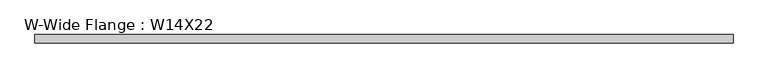
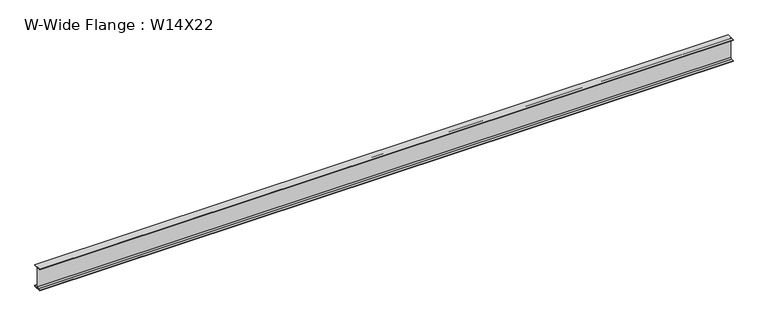
"""IFC4 building model written with IfcOpenShell, lengths in millimetres: beam geometry, W-Wide Flange : W14X22."""

import ifcopenshell
import ifcopenshell.guid

model = None  # the IFC model being written
_history = None  # IfcOwnerHistory: only IFC2X3 demands one
_inside = {}  # id of a spatial element -> (the spatial element, [elements in it])
_under = {}  # id of a project, library or spatial element -> (it, [spatial elements below it])
_declared = {}  # id of a project -> (the project, [libraries it declares])
_typed = {}  # id of a type object -> (the type object, [elements of that type])
_made_of = {}  # id of a material, layer set ... -> (it, [elements and type objects made of it])


def new_model(schema):
    """Start an empty IFC model of exactly this schema.

    Asked for "IFC4X3", IfcOpenShell would pick the latest addendum, in which some entities
    have other attributes; the version numbers below select the first issue.
    IFC2X3 requires an IfcOwnerHistory on every rooted entity: one is made here for all.
    """
    global model, _history
    if schema == "IFC4X3":
        model = ifcopenshell.file(schema_version=(4, 3, 0, 0))
    else:
        model = ifcopenshell.file(schema=schema)
    _inside.clear()
    _under.clear()
    _declared.clear()
    _typed.clear()
    _made_of.clear()
    _history = None
    if model.schema == "IFC2X3":
        org = make("IfcOrganization", Name="unknown")
        user = make(
            "IfcPersonAndOrganization",
            ThePerson=make("IfcPerson", FamilyName="unknown"),
            TheOrganization=org,
        )
        app = make(
            "IfcApplication",
            ApplicationDeveloper=org,
            Version="unknown",
            ApplicationFullName="unknown",
            ApplicationIdentifier="unknown",
        )
        _history = make(
            "IfcOwnerHistory",
            OwningUser=user,
            OwningApplication=app,
            ChangeAction="ADDED",
            CreationDate=0,
        )
    return model


def make(cls, **values):
    """One entity of the class cls with the attributes given. An attribute that is None is left unset."""
    return model.create_entity(
        cls, **{name: value for name, value in values.items() if value is not None}
    )


def rooted(cls, **values):
    """An entity with a GlobalId (a new one), such as an element, a storey or a relation."""
    return make(cls, GlobalId=ifcopenshell.guid.new(), OwnerHistory=_history, **values)


def si_unit(unit_type, name, prefix=None):
    """IfcSIUnit, for example si_unit("LENGTHUNIT", "METRE", prefix="MILLI")."""
    return make("IfcSIUnit", UnitType=unit_type, Prefix=prefix, Name=name)


def assignment(units):
    """IfcUnitAssignment: the units of a project."""
    return None if units is None else make("IfcUnitAssignment", Units=units)


def point(xyz):
    """IfcCartesianPoint."""
    return None if xyz is None else make("IfcCartesianPoint", Coordinates=xyz)


def direction(xyz):
    """IfcDirection."""
    return None if xyz is None else make("IfcDirection", DirectionRatios=xyz)


def frame(location, z_axis=None, x_axis=None):
    """IfcAxis2Placement3D, a coordinate frame: its origin and axes. An axis left out is left unset."""
    return make(
        "IfcAxis2Placement3D",
        Location=point(location),
        Axis=direction(z_axis),
        RefDirection=direction(x_axis),
    )


def frame_2d(location, x_axis=None):
    """IfcAxis2Placement2D, a coordinate frame in the plane: its origin and x axis."""
    return make(
        "IfcAxis2Placement2D", Location=point(location), RefDirection=direction(x_axis)
    )


def origin():
    """The frame at (0, 0, 0) with its axes left unset."""
    return frame((0.0, 0.0, 0.0))


def place(relative_to, where):
    """IfcLocalPlacement: puts the frame where relative to a parent placement (None: the world)."""
    return make(
        "IfcLocalPlacement", PlacementRelTo=relative_to, RelativePlacement=where
    )


def context(
    kind, dimensions, precision=None, world=None, true_north=None, identifier=None
):
    """IfcGeometricRepresentationContext, for example the 3D "Model" context."""
    return make(
        "IfcGeometricRepresentationContext",
        ContextIdentifier=identifier,
        ContextType=kind,
        CoordinateSpaceDimension=dimensions,
        Precision=precision,
        WorldCoordinateSystem=world,
        TrueNorth=true_north,
    )


def project(units=None, contexts=None):
    """IfcProject with its units and contexts."""
    return rooted(
        "IfcProject",
        Name="project",
        RepresentationContexts=contexts,
        UnitsInContext=assignment(units),
    )


def spatial(cls, under=None, at=None, **own):
    """A site, building, storey or space (cls), placed at a placement, below another one or the project."""
    s = rooted(cls, ObjectPlacement=at, **own)
    if under is not None:
        _under.setdefault(under.id(), (under, []))[1].append(s)
    return s


def polyline(points):
    """IfcPolyline through the points."""
    return make("IfcPolyline", Points=[point(p) for p in points])


def circle_curve(where, radius):
    """IfcCircle in the frame where."""
    return make("IfcCircle", Position=where, Radius=radius)


def trimmed(basis, trim1, trim2, sense, master):
    """IfcTrimmedCurve: the piece of a basis curve between two trims."""
    return make(
        "IfcTrimmedCurve",
        BasisCurve=basis,
        Trim1=trim1,
        Trim2=trim2,
        SenseAgreement=sense,
        MasterRepresentation=master,
    )


def segment(curve, same_sense, transition):
    """IfcCompositeCurveSegment."""
    return make(
        "IfcCompositeCurveSegment",
        Transition=transition,
        SameSense=same_sense,
        ParentCurve=curve,
    )


def composite_curve(segments, self_intersect=None):
    """IfcCompositeCurve: segments joined end to end."""
    return make("IfcCompositeCurve", Segments=segments, SelfIntersect=self_intersect)


def outline(outer, holes=None, kind="AREA"):
    """IfcArbitraryClosedProfileDef: a profile drawn as a closed curve; with holes, ...WithVoids."""
    if holes is None:
        return make("IfcArbitraryClosedProfileDef", ProfileType=kind, OuterCurve=outer)
    return make(
        "IfcArbitraryProfileDefWithVoids",
        ProfileType=kind,
        OuterCurve=outer,
        InnerCurves=holes,
    )


def extrude(swept, where, along, depth):
    """IfcExtrudedAreaSolid: the profile swept, set in the frame where, extruded along a direction by depth."""
    return make(
        "IfcExtrudedAreaSolid",
        SweptArea=swept,
        Position=where,
        ExtrudedDirection=direction(along),
        Depth=depth,
    )


def shape(context_of_items, identifier, shape_type, items):
    """IfcShapeRepresentation: the items that make up one representation, for example the "Body"."""
    return make(
        "IfcShapeRepresentation",
        ContextOfItems=context_of_items,
        RepresentationIdentifier=identifier,
        RepresentationType=shape_type,
        Items=items,
    )


def source(mapping_origin, context_of_items, identifier, shape_type, items):
    """IfcRepresentationMap: a shape defined once, which mapped items show again and again."""
    return make(
        "IfcRepresentationMap",
        MappingOrigin=mapping_origin,
        MappedRepresentation=shape(context_of_items, identifier, shape_type, items),
    )


def transform(
    local_origin,
    x_axis=None,
    y_axis=None,
    z_axis=None,
    scale=None,
    scale2=None,
    scale3=None,
    uniform=True,
):
    """IfcCartesianTransformationOperator3D, or its non-uniform kind. x_axis, y_axis, z_axis: its Axis1, 2, 3."""
    if uniform:
        return make(
            "IfcCartesianTransformationOperator3D",
            Axis1=direction(x_axis),
            Axis2=direction(y_axis),
            LocalOrigin=point(local_origin),
            Scale=scale,
            Axis3=direction(z_axis),
        )
    return make(
        "IfcCartesianTransformationOperator3DnonUniform",
        Axis1=direction(x_axis),
        Axis2=direction(y_axis),
        LocalOrigin=point(local_origin),
        Scale=scale,
        Axis3=direction(z_axis),
        Scale2=scale2,
        Scale3=scale3,
    )


def mapped(mapping_source, mapping_target):
    """IfcMappedItem: shows the shape of a source again, moved by a transform."""
    return make(
        "IfcMappedItem", MappingSource=mapping_source, MappingTarget=mapping_target
    )


def made_of(thing, what):
    """Note that an element or type object is made of a material, layer set ...; save() writes the relation."""
    if what is not None:
        _made_of.setdefault(what.id(), (what, []))[1].append(thing)
    return thing


def element(
    cls,
    number,
    at=None,
    inside=None,
    cuts=None,
    type_object=None,
    material=None,
    context=None,
    identifier="Body",
    shape_type=None,
    held_by="IfcProductDefinitionShape",
    body=None,
    shapes=None,
    **own,
):
    """One element of the class cls, such as IfcWall. Its Tag is "e" and its number.

    at: its placement. inside: the storey or other place that contains it. cuts: it is an
    opening in that element (IfcRelVoidsElement). A single representation is given by context,
    identifier, shape_type and body (its items); several are given by shapes. held_by: the class
    of the entity that holds the representations. save() writes the other relations.
    """
    e = rooted(cls, Tag="e%d" % number, ObjectPlacement=at, **own)
    if body is not None:
        shapes = [shape(context, identifier, shape_type, body)]
    if shapes is not None:
        e.Representation = make(held_by, Representations=shapes)
    if inside is not None:
        _inside.setdefault(inside.id(), (inside, []))[1].append(e)
    if cuts is not None:
        rooted(
            "IfcRelVoidsElement", RelatingBuildingElement=cuts, RelatedOpeningElement=e
        )
    if type_object is not None:
        _typed.setdefault(type_object.id(), (type_object, []))[1].append(e)
    return made_of(e, material)


def aggregate(whole, parts):
    """IfcRelAggregates: a whole, such as a stair, and the parts it consists of."""
    return rooted("IfcRelAggregates", RelatingObject=whole, RelatedObjects=parts)


def save(model, path):
    """Write the relations noted so far, then the file.

    IfcRelAggregates (storeys below a building ...), IfcRelContainedInSpatialStructure (elements
    in a storey), IfcRelDefinesByType, IfcRelAssociatesMaterial and IfcRelDeclares: one each for
    every whole, place, type object, material and project.
    """
    for whole, parts in _under.values():
        aggregate(whole, parts)
    for where, things in _inside.values():
        rooted(
            "IfcRelContainedInSpatialStructure",
            RelatedElements=things,
            RelatingStructure=where,
        )
    for kind, things in _typed.values():
        rooted("IfcRelDefinesByType", RelatedObjects=things, RelatingType=kind)
    for what, things in _made_of.values():
        rooted("IfcRelAssociatesMaterial", RelatedObjects=things, RelatingMaterial=what)
    for by, libraries in _declared.values():
        rooted("IfcRelDeclares", RelatingContext=by, RelatedDefinitions=libraries)
    model.write(path)


def w_wide_flange_w14x22_9d42d0bf(model_context):
    return source(origin(), model_context, "Body", "SweptSolid", [
        extrude(outline(composite_curve([segment(polyline([(63.5, -165.481), (63.5, -173.99), (-63.5, -173.99), (-63.5, -165.481), (-21.3995, -165.481)]), True, "CONTINUOUS"), segment(trimmed(circle_curve(frame_2d((-21.3995, -147.0025)), 18.4785), [point((-21.3995, -165.481))], [point((-2.921, -147.0025))], True, "CARTESIAN"), True, "CONTINUOUS"), segment(polyline([(-2.921, -147.0025), (-2.921, 147.0025)]), True, "CONTINUOUS"), segment(trimmed(circle_curve(frame_2d((-21.3995, 147.0025)), 18.4785), [point((-2.921, 147.0025))], [point((-21.3995, 165.481))], True, "CARTESIAN"), True, "CONTINUOUS"), segment(polyline([(-21.3995, 165.481), (-63.5, 165.481), (-63.5, 173.99), (63.5, 173.99), (63.5, 165.481), (21.3995, 165.481)]), True, "CONTINUOUS"), segment(trimmed(circle_curve(frame_2d((21.3995, 147.0025)), 18.4785), [point((21.3995, 165.481))], [point((2.921, 147.0025))], True, "CARTESIAN"), True, "CONTINUOUS"), segment(polyline([(2.921, 147.0025), (2.921, -147.0025)]), True, "CONTINUOUS"), segment(trimmed(circle_curve(frame_2d((21.3995, -147.0025)), 18.4785), [point((2.921, -147.0025))], [point((21.3995, -165.481))], True, "CARTESIAN"), True, "CONTINUOUS"), segment(polyline([(21.3995, -165.481), (63.5, -165.481)]), True, "CONTINUOUS")], self_intersect=False)), frame((-5367.4041564, 0.0, 0.0), z_axis=(1.0, 0.0, 0.0), x_axis=(0.0, 1.0, 0.0)), (0.0, 0.0, 1.0), 10624.6462147),
    ])


if __name__ == "__main__":
    model = new_model("IFC4")
    model_context = context("Model", 3, world=origin())
    ifc_project = project(units=[si_unit("LENGTHUNIT", "METRE", prefix="MILLI")], contexts=[model_context])
    site = spatial("IfcSite", under=ifc_project)
    building = spatial("IfcBuilding", under=site)
    placement = place(None, origin())
    w_wide_flange_w14x22_shape = w_wide_flange_w14x22_9d42d0bf(model_context)
    element("IfcBeam", 1, ObjectType="W-Wide Flange : W14X22", at=placement, inside=building, context=model_context, shape_type="MappedRepresentation", body=[
        mapped(w_wide_flange_w14x22_shape, transform((0.0, 0.0, 0.0), x_axis=(1.0, 0.0, 0.0), y_axis=(0.0, 1.0, 0.0), z_axis=(0.0, 0.0, 1.0))),
    ])
    save(model, "model.ifc")

# Revit data of these elements
# Type "W-Wide Flange : W14X22"
#   Assembly Code = "B10"
#   W = 22
#   Length [instance default] = 5' - 0"
#   bf = 0' - 5"
#   d = 1' - 1.7"
#   k = 0' - 1 1/16"
#   k2 = 0' - 0.7275"
#   tf = 0' - 0.335"
#   tw = 0' - 0.23"
#   A = 0.0450694 SF
#   Structural Material [instance default] = Steel ASTM A992
# Element 1 (IfcBeam, "W-Wide Flange : W14X22")
#   Structural Material = STRUCTURAL STEEL - SEE STRUCT. DWGS
#   Materials on its faces: "STRUCTURAL STEEL - SEE STRUCT. DWGS"
# Materials
#   "Steel ASTM A992": class "Metal", colour RGB 199 199 199, transparency 0, Description = "Structural steel 50ksi", Cost = 0
#   "STRUCTURAL STEEL - SEE STRUCT. DWGS": class "Metal", colour RGB 137 146 153, transparency 0, Description = "Steel, mill finish", Cost = 0
